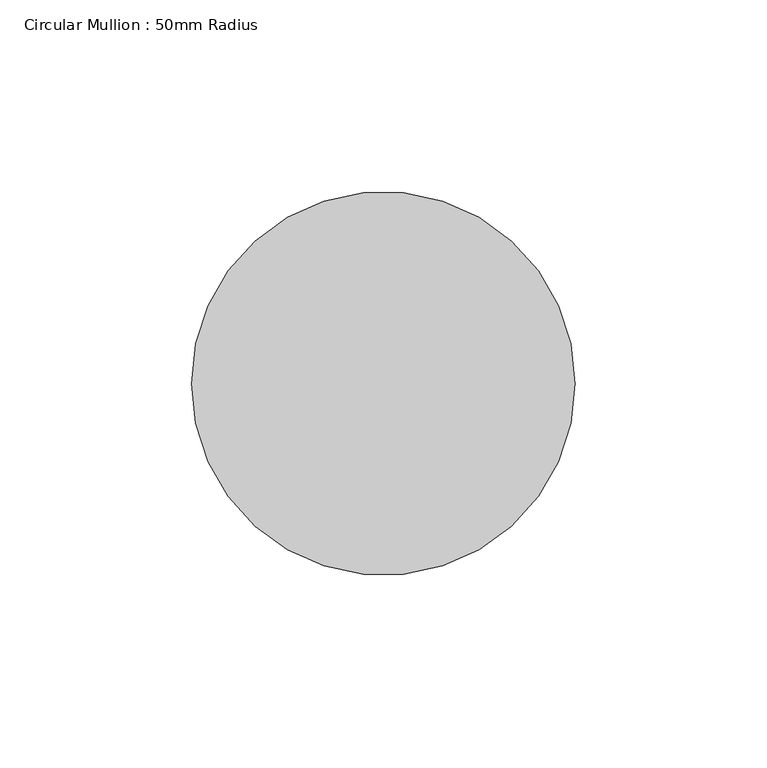
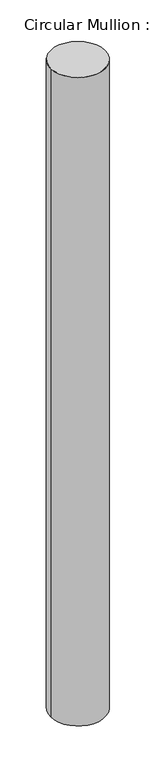
"""IFC4 building model written with IfcOpenShell, lengths in millimetres: member geometry, Circular Mullion : 50mm Radius."""

import ifcopenshell
import ifcopenshell.guid

model = None  # the IFC model being written
_history = None  # IfcOwnerHistory: only IFC2X3 demands one
_inside = {}  # id of a spatial element -> (the spatial element, [elements in it])
_under = {}  # id of a project, library or spatial element -> (it, [spatial elements below it])
_declared = {}  # id of a project -> (the project, [libraries it declares])
_typed = {}  # id of a type object -> (the type object, [elements of that type])
_made_of = {}  # id of a material, layer set ... -> (it, [elements and type objects made of it])


def new_model(schema):
    """Start an empty IFC model of exactly this schema.

    Asked for "IFC4X3", IfcOpenShell would pick the latest addendum, in which some entities
    have other attributes; the version numbers below select the first issue.
    IFC2X3 requires an IfcOwnerHistory on every rooted entity: one is made here for all.
    """
    global model, _history
    if schema == "IFC4X3":
        model = ifcopenshell.file(schema_version=(4, 3, 0, 0))
    else:
        model = ifcopenshell.file(schema=schema)
    _inside.clear()
    _under.clear()
    _declared.clear()
    _typed.clear()
    _made_of.clear()
    _history = None
    if model.schema == "IFC2X3":
        org = make("IfcOrganization", Name="unknown")
        user = make(
            "IfcPersonAndOrganization",
            ThePerson=make("IfcPerson", FamilyName="unknown"),
            TheOrganization=org,
        )
        app = make(
            "IfcApplication",
            ApplicationDeveloper=org,
            Version="unknown",
            ApplicationFullName="unknown",
            ApplicationIdentifier="unknown",
        )
        _history = make(
            "IfcOwnerHistory",
            OwningUser=user,
            OwningApplication=app,
            ChangeAction="ADDED",
            CreationDate=0,
        )
    return model


def make(cls, **values):
    """One entity of the class cls with the attributes given. An attribute that is None is left unset."""
    return model.create_entity(
        cls, **{name: value for name, value in values.items() if value is not None}
    )


def rooted(cls, **values):
    """An entity with a GlobalId (a new one), such as an element, a storey or a relation."""
    return make(cls, GlobalId=ifcopenshell.guid.new(), OwnerHistory=_history, **values)


def si_unit(unit_type, name, prefix=None):
    """IfcSIUnit, for example si_unit("LENGTHUNIT", "METRE", prefix="MILLI")."""
    return make("IfcSIUnit", UnitType=unit_type, Prefix=prefix, Name=name)


def assignment(units):
    """IfcUnitAssignment: the units of a project."""
    return None if units is None else make("IfcUnitAssignment", Units=units)


def point(xyz):
    """IfcCartesianPoint."""
    return None if xyz is None else make("IfcCartesianPoint", Coordinates=xyz)


def direction(xyz):
    """IfcDirection."""
    return None if xyz is None else make("IfcDirection", DirectionRatios=xyz)


def frame(location, z_axis=None, x_axis=None):
    """IfcAxis2Placement3D, a coordinate frame: its origin and axes. An axis left out is left unset."""
    return make(
        "IfcAxis2Placement3D",
        Location=point(location),
        Axis=direction(z_axis),
        RefDirection=direction(x_axis),
    )


def frame_2d(location, x_axis=None):
    """IfcAxis2Placement2D, a coordinate frame in the plane: its origin and x axis."""
    return make(
        "IfcAxis2Placement2D", Location=point(location), RefDirection=direction(x_axis)
    )


def origin():
    """The frame at (0, 0, 0) with its axes left unset."""
    return frame((0.0, 0.0, 0.0))


def origin_2d():
    """The frame at (0, 0) in the plane with its x axis left unset."""
    return frame_2d((0.0, 0.0))


def place(relative_to, where):
    """IfcLocalPlacement: puts the frame where relative to a parent placement (None: the world)."""
    return make(
        "IfcLocalPlacement", PlacementRelTo=relative_to, RelativePlacement=where
    )


def context(
    kind, dimensions, precision=None, world=None, true_north=None, identifier=None
):
    """IfcGeometricRepresentationContext, for example the 3D "Model" context."""
    return make(
        "IfcGeometricRepresentationContext",
        ContextIdentifier=identifier,
        ContextType=kind,
        CoordinateSpaceDimension=dimensions,
        Precision=precision,
        WorldCoordinateSystem=world,
        TrueNorth=true_north,
    )


def project(units=None, contexts=None):
    """IfcProject with its units and contexts."""
    return rooted(
        "IfcProject",
        Name="project",
        RepresentationContexts=contexts,
        UnitsInContext=assignment(units),
    )


def spatial(cls, under=None, at=None, **own):
    """A site, building, storey or space (cls), placed at a placement, below another one or the project."""
    s = rooted(cls, ObjectPlacement=at, **own)
    if under is not None:
        _under.setdefault(under.id(), (under, []))[1].append(s)
    return s


def circle_curve(where, radius):
    """IfcCircle in the frame where."""
    return make("IfcCircle", Position=where, Radius=radius)


def trimmed(basis, trim1, trim2, sense, master):
    """IfcTrimmedCurve: the piece of a basis curve between two trims."""
    return make(
        "IfcTrimmedCurve",
        BasisCurve=basis,
        Trim1=trim1,
        Trim2=trim2,
        SenseAgreement=sense,
        MasterRepresentation=master,
    )


def segment(curve, same_sense, transition):
    """IfcCompositeCurveSegment."""
    return make(
        "IfcCompositeCurveSegment",
        Transition=transition,
        SameSense=same_sense,
        ParentCurve=curve,
    )


def composite_curve(segments, self_intersect=None):
    """IfcCompositeCurve: segments joined end to end."""
    return make("IfcCompositeCurve", Segments=segments, SelfIntersect=self_intersect)


def outline(outer, holes=None, kind="AREA"):
    """IfcArbitraryClosedProfileDef: a profile drawn as a closed curve; with holes, ...WithVoids."""
    if holes is None:
        return make("IfcArbitraryClosedProfileDef", ProfileType=kind, OuterCurve=outer)
    return make(
        "IfcArbitraryProfileDefWithVoids",
        ProfileType=kind,
        OuterCurve=outer,
        InnerCurves=holes,
    )


def extrude(swept, where, along, depth):
    """IfcExtrudedAreaSolid: the profile swept, set in the frame where, extruded along a direction by depth."""
    return make(
        "IfcExtrudedAreaSolid",
        SweptArea=swept,
        Position=where,
        ExtrudedDirection=direction(along),
        Depth=depth,
    )


def shape(context_of_items, identifier, shape_type, items):
    """IfcShapeRepresentation: the items that make up one representation, for example the "Body"."""
    return make(
        "IfcShapeRepresentation",
        ContextOfItems=context_of_items,
        RepresentationIdentifier=identifier,
        RepresentationType=shape_type,
        Items=items,
    )


def source(mapping_origin, context_of_items, identifier, shape_type, items):
    """IfcRepresentationMap: a shape defined once, which mapped items show again and again."""
    return make(
        "IfcRepresentationMap",
        MappingOrigin=mapping_origin,
        MappedRepresentation=shape(context_of_items, identifier, shape_type, items),
    )


def transform(
    local_origin,
    x_axis=None,
    y_axis=None,
    z_axis=None,
    scale=None,
    scale2=None,
    scale3=None,
    uniform=True,
):
    """IfcCartesianTransformationOperator3D, or its non-uniform kind. x_axis, y_axis, z_axis: its Axis1, 2, 3."""
    if uniform:
        return make(
            "IfcCartesianTransformationOperator3D",
            Axis1=direction(x_axis),
            Axis2=direction(y_axis),
            LocalOrigin=point(local_origin),
            Scale=scale,
            Axis3=direction(z_axis),
        )
    return make(
        "IfcCartesianTransformationOperator3DnonUniform",
        Axis1=direction(x_axis),
        Axis2=direction(y_axis),
        LocalOrigin=point(local_origin),
        Scale=scale,
        Axis3=direction(z_axis),
        Scale2=scale2,
        Scale3=scale3,
    )


def mapped(mapping_source, mapping_target):
    """IfcMappedItem: shows the shape of a source again, moved by a transform."""
    return make(
        "IfcMappedItem", MappingSource=mapping_source, MappingTarget=mapping_target
    )


def made_of(thing, what):
    """Note that an element or type object is made of a material, layer set ...; save() writes the relation."""
    if what is not None:
        _made_of.setdefault(what.id(), (what, []))[1].append(thing)
    return thing


def element(
    cls,
    number,
    at=None,
    inside=None,
    cuts=None,
    type_object=None,
    material=None,
    context=None,
    identifier="Body",
    shape_type=None,
    held_by="IfcProductDefinitionShape",
    body=None,
    shapes=None,
    **own,
):
    """One element of the class cls, such as IfcWall. Its Tag is "e" and its number.

    at: its placement. inside: the storey or other place that contains it. cuts: it is an
    opening in that element (IfcRelVoidsElement). A single representation is given by context,
    identifier, shape_type and body (its items); several are given by shapes. held_by: the class
    of the entity that holds the representations. save() writes the other relations.
    """
    e = rooted(cls, Tag="e%d" % number, ObjectPlacement=at, **own)
    if body is not None:
        shapes = [shape(context, identifier, shape_type, body)]
    if shapes is not None:
        e.Representation = make(held_by, Representations=shapes)
    if inside is not None:
        _inside.setdefault(inside.id(), (inside, []))[1].append(e)
    if cuts is not None:
        rooted(
            "IfcRelVoidsElement", RelatingBuildingElement=cuts, RelatedOpeningElement=e
        )
    if type_object is not None:
        _typed.setdefault(type_object.id(), (type_object, []))[1].append(e)
    return made_of(e, material)


def aggregate(whole, parts):
    """IfcRelAggregates: a whole, such as a stair, and the parts it consists of."""
    return rooted("IfcRelAggregates", RelatingObject=whole, RelatedObjects=parts)


def save(model, path):
    """Write the relations noted so far, then the file.

    IfcRelAggregates (storeys below a building ...), IfcRelContainedInSpatialStructure (elements
    in a storey), IfcRelDefinesByType, IfcRelAssociatesMaterial and IfcRelDeclares: one each for
    every whole, place, type object, material and project.
    """
    for whole, parts in _under.values():
        aggregate(whole, parts)
    for where, things in _inside.values():
        rooted(
            "IfcRelContainedInSpatialStructure",
            RelatedElements=things,
            RelatingStructure=where,
        )
    for kind, things in _typed.values():
        rooted("IfcRelDefinesByType", RelatedObjects=things, RelatingType=kind)
    for what, things in _made_of.values():
        rooted("IfcRelAssociatesMaterial", RelatedObjects=things, RelatingMaterial=what)
    for by, libraries in _declared.values():
        rooted("IfcRelDeclares", RelatingContext=by, RelatedDefinitions=libraries)
    model.write(path)


def circular_mullion_50mm_radius_fb57abd5(model_context):
    return source(origin(), model_context, "Body", "SweptSolid", [
        extrude(outline(composite_curve([segment(trimmed(circle_curve(origin_2d(), 50.0), [point((50.0, 0.0))], [point((-50.0, 0.0))], False, "CARTESIAN"), True, "CONTINUOUS"), segment(trimmed(circle_curve(origin_2d(), 50.0), [point((-50.0, 0.0))], [point((50.0, 0.0))], False, "CARTESIAN"), True, "CONTINUOUS")], self_intersect=False)), frame((0.0, 0.0, -1260.8692397), z_axis=(0.0, 0.0, 1.0), x_axis=(1.0, 0.0, 0.0)), (0.0, 0.0, 1.0), 1260.8692397),
    ])


if __name__ == "__main__":
    model = new_model("IFC4")
    model_context = context("Model", 3, world=origin())
    ifc_project = project(units=[si_unit("LENGTHUNIT", "METRE", prefix="MILLI")], contexts=[model_context])
    site = spatial("IfcSite", under=ifc_project)
    building = spatial("IfcBuilding", under=site)
    placement = place(None, origin())
    circular_mullion_50mm_radius_shape = circular_mullion_50mm_radius_fb57abd5(model_context)
    element("IfcMember", 1, ObjectType="Circular Mullion : 50mm Radius", at=placement, inside=building, context=model_context, shape_type="MappedRepresentation", body=[
        mapped(circular_mullion_50mm_radius_shape, transform((0.0, 0.0, 0.0), x_axis=(1.0, 0.0, 0.0), y_axis=(0.0, 1.0, 0.0), z_axis=(0.0, 0.0, 1.0))),
    ])
    save(model, "model.ifc")

# Revit data of these elements
# Type "Circular Mullion : 50mm Radius"
#   built-in parameter 1007350 = 0.164042 (stored number, unit not read)
# Element 1 (IfcMember, "Circular Mullion : 50mm Radius")
#   Materials on its faces: "Aluminium"
# Materials
#   "Aluminium": class "Metal", colour RGB 247 247 247, transparency 0, Description = "Aluminium 6061", Cost = 0
